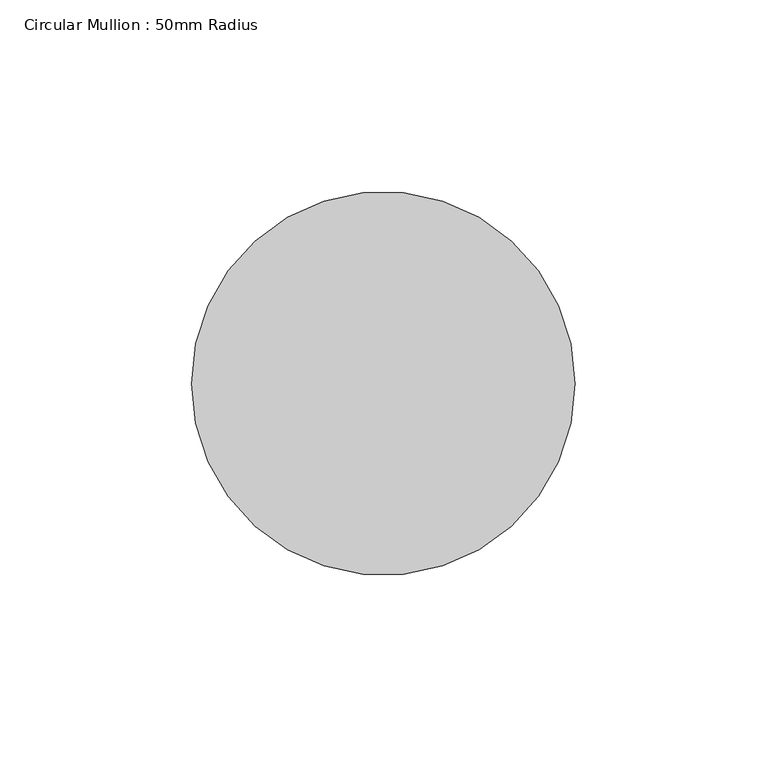
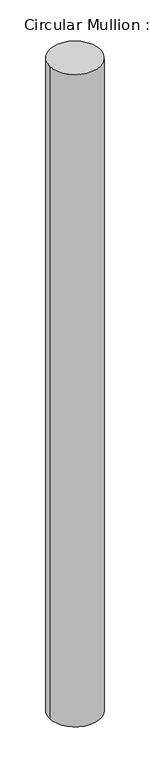
"""IFC4 building model written with IfcOpenShell, lengths in millimetres: member geometry, Circular Mullion : 50mm Radius."""

import ifcopenshell
import ifcopenshell.guid

model = None  # the IFC model being written
_history = None  # IfcOwnerHistory: only IFC2X3 demands one
_inside = {}  # id of a spatial element -> (the spatial element, [elements in it])
_under = {}  # id of a project, library or spatial element -> (it, [spatial elements below it])
_declared = {}  # id of a project -> (the project, [libraries it declares])
_typed = {}  # id of a type object -> (the type object, [elements of that type])
_made_of = {}  # id of a material, layer set ... -> (it, [elements and type objects made of it])


def new_model(schema):
    """Start an empty IFC model of exactly this schema.

    Asked for "IFC4X3", IfcOpenShell would pick the latest addendum, in which some entities
    have other attributes; the version numbers below select the first issue.
    IFC2X3 requires an IfcOwnerHistory on every rooted entity: one is made here for all.
    """
    global model, _history
    if schema == "IFC4X3":
        model = ifcopenshell.file(schema_version=(4, 3, 0, 0))
    else:
        model = ifcopenshell.file(schema=schema)
    _inside.clear()
    _under.clear()
    _declared.clear()
    _typed.clear()
    _made_of.clear()
    _history = None
    if model.schema == "IFC2X3":
        org = make("IfcOrganization", Name="unknown")
        user = make(
            "IfcPersonAndOrganization",
            ThePerson=make("IfcPerson", FamilyName="unknown"),
            TheOrganization=org,
        )
        app = make(
            "IfcApplication",
            ApplicationDeveloper=org,
            Version="unknown",
            ApplicationFullName="unknown",
            ApplicationIdentifier="unknown",
        )
        _history = make(
            "IfcOwnerHistory",
            OwningUser=user,
            OwningApplication=app,
            ChangeAction="ADDED",
            CreationDate=0,
        )
    return model


def make(cls, **values):
    """One entity of the class cls with the attributes given. An attribute that is None is left unset."""
    return model.create_entity(
        cls, **{name: value for name, value in values.items() if value is not None}
    )


def rooted(cls, **values):
    """An entity with a GlobalId (a new one), such as an element, a storey or a relation."""
    return make(cls, GlobalId=ifcopenshell.guid.new(), OwnerHistory=_history, **values)


def si_unit(unit_type, name, prefix=None):
    """IfcSIUnit, for example si_unit("LENGTHUNIT", "METRE", prefix="MILLI")."""
    return make("IfcSIUnit", UnitType=unit_type, Prefix=prefix, Name=name)


def assignment(units):
    """IfcUnitAssignment: the units of a project."""
    return None if units is None else make("IfcUnitAssignment", Units=units)


def point(xyz):
    """IfcCartesianPoint."""
    return None if xyz is None else make("IfcCartesianPoint", Coordinates=xyz)


def direction(xyz):
    """IfcDirection."""
    return None if xyz is None else make("IfcDirection", DirectionRatios=xyz)


def frame(location, z_axis=None, x_axis=None):
    """IfcAxis2Placement3D, a coordinate frame: its origin and axes. An axis left out is left unset."""
    return make(
        "IfcAxis2Placement3D",
        Location=point(location),
        Axis=direction(z_axis),
        RefDirection=direction(x_axis),
    )


def frame_2d(location, x_axis=None):
    """IfcAxis2Placement2D, a coordinate frame in the plane: its origin and x axis."""
    return make(
        "IfcAxis2Placement2D", Location=point(location), RefDirection=direction(x_axis)
    )


def origin():
    """The frame at (0, 0, 0) with its axes left unset."""
    return frame((0.0, 0.0, 0.0))


def origin_2d():
    """The frame at (0, 0) in the plane with its x axis left unset."""
    return frame_2d((0.0, 0.0))


def place(relative_to, where):
    """IfcLocalPlacement: puts the frame where relative to a parent placement (None: the world)."""
    return make(
        "IfcLocalPlacement", PlacementRelTo=relative_to, RelativePlacement=where
    )


def context(
    kind, dimensions, precision=None, world=None, true_north=None, identifier=None
):
    """IfcGeometricRepresentationContext, for example the 3D "Model" context."""
    return make(
        "IfcGeometricRepresentationContext",
        ContextIdentifier=identifier,
        ContextType=kind,
        CoordinateSpaceDimension=dimensions,
        Precision=precision,
        WorldCoordinateSystem=world,
        TrueNorth=true_north,
    )


def project(units=None, contexts=None):
    """IfcProject with its units and contexts."""
    return rooted(
        "IfcProject",
        Name="project",
        RepresentationContexts=contexts,
        UnitsInContext=assignment(units),
    )


def spatial(cls, under=None, at=None, **own):
    """A site, building, storey or space (cls), placed at a placement, below another one or the project."""
    s = rooted(cls, ObjectPlacement=at, **own)
    if under is not None:
        _under.setdefault(under.id(), (under, []))[1].append(s)
    return s


def circle_curve(where, radius):
    """IfcCircle in the frame where."""
    return make("IfcCircle", Position=where, Radius=radius)


def trimmed(basis, trim1, trim2, sense, master):
    """IfcTrimmedCurve: the piece of a basis curve between two trims."""
    return make(
        "IfcTrimmedCurve",
        BasisCurve=basis,
        Trim1=trim1,
        Trim2=trim2,
        SenseAgreement=sense,
        MasterRepresentation=master,
    )


def segment(curve, same_sense, transition):
    """IfcCompositeCurveSegment."""
    return make(
        "IfcCompositeCurveSegment",
        Transition=transition,
        SameSense=same_sense,
        ParentCurve=curve,
    )


def composite_curve(segments, self_intersect=None):
    """IfcCompositeCurve: segments joined end to end."""
    return make("IfcCompositeCurve", Segments=segments, SelfIntersect=self_intersect)


def outline(outer, holes=None, kind="AREA"):
    """IfcArbitraryClosedProfileDef: a profile drawn as a closed curve; with holes, ...WithVoids."""
    if holes is None:
        return make("IfcArbitraryClosedProfileDef", ProfileType=kind, OuterCurve=outer)
    return make(
        "IfcArbitraryProfileDefWithVoids",
        ProfileType=kind,
        OuterCurve=outer,
        InnerCurves=holes,
    )


def extrude(swept, where, along, depth):
    """IfcExtrudedAreaSolid: the profile swept, set in the frame where, extruded along a direction by depth."""
    return make(
        "IfcExtrudedAreaSolid",
        SweptArea=swept,
        Position=where,
        ExtrudedDirection=direction(along),
        Depth=depth,
    )


def shape(context_of_items, identifier, shape_type, items):
    """IfcShapeRepresentation: the items that make up one representation, for example the "Body"."""
    return make(
        "IfcShapeRepresentation",
        ContextOfItems=context_of_items,
        RepresentationIdentifier=identifier,
        RepresentationType=shape_type,
        Items=items,
    )


def source(mapping_origin, context_of_items, identifier, shape_type, items):
    """IfcRepresentationMap: a shape defined once, which mapped items show again and again."""
    return make(
        "IfcRepresentationMap",
        MappingOrigin=mapping_origin,
        MappedRepresentation=shape(context_of_items, identifier, shape_type, items),
    )


def transform(
    local_origin,
    x_axis=None,
    y_axis=None,
    z_axis=None,
    scale=None,
    scale2=None,
    scale3=None,
    uniform=True,
):
    """IfcCartesianTransformationOperator3D, or its non-uniform kind. x_axis, y_axis, z_axis: its Axis1, 2, 3."""
    if uniform:
        return make(
            "IfcCartesianTransformationOperator3D",
            Axis1=direction(x_axis),
            Axis2=direction(y_axis),
            LocalOrigin=point(local_origin),
            Scale=scale,
            Axis3=direction(z_axis),
        )
    return make(
        "IfcCartesianTransformationOperator3DnonUniform",
        Axis1=direction(x_axis),
        Axis2=direction(y_axis),
        LocalOrigin=point(local_origin),
        Scale=scale,
        Axis3=direction(z_axis),
        Scale2=scale2,
        Scale3=scale3,
    )


def mapped(mapping_source, mapping_target):
    """IfcMappedItem: shows the shape of a source again, moved by a transform."""
    return make(
        "IfcMappedItem", MappingSource=mapping_source, MappingTarget=mapping_target
    )


def made_of(thing, what):
    """Note that an element or type object is made of a material, layer set ...; save() writes the relation."""
    if what is not None:
        _made_of.setdefault(what.id(), (what, []))[1].append(thing)
    return thing


def element(
    cls,
    number,
    at=None,
    inside=None,
    cuts=None,
    type_object=None,
    material=None,
    context=None,
    identifier="Body",
    shape_type=None,
    held_by="IfcProductDefinitionShape",
    body=None,
    shapes=None,
    **own,
):
    """One element of the class cls, such as IfcWall. Its Tag is "e" and its number.

    at: its placement. inside: the storey or other place that contains it. cuts: it is an
    opening in that element (IfcRelVoidsElement). A single representation is given by context,
    identifier, shape_type and body (its items); several are given by shapes. held_by: the class
    of the entity that holds the representations. save() writes the other relations.
    """
    e = rooted(cls, Tag="e%d" % number, ObjectPlacement=at, **own)
    if body is not None:
        shapes = [shape(context, identifier, shape_type, body)]
    if shapes is not None:
        e.Representation = make(held_by, Representations=shapes)
    if inside is not None:
        _inside.setdefault(inside.id(), (inside, []))[1].append(e)
    if cuts is not None:
        rooted(
            "IfcRelVoidsElement", RelatingBuildingElement=cuts, RelatedOpeningElement=e
        )
    if type_object is not None:
        _typed.setdefault(type_object.id(), (type_object, []))[1].append(e)
    return made_of(e, material)


def aggregate(whole, parts):
    """IfcRelAggregates: a whole, such as a stair, and the parts it consists of."""
    return rooted("IfcRelAggregates", RelatingObject=whole, RelatedObjects=parts)


def save(model, path):
    """Write the relations noted so far, then the file.

    IfcRelAggregates (storeys below a building ...), IfcRelContainedInSpatialStructure (elements
    in a storey), IfcRelDefinesByType, IfcRelAssociatesMaterial and IfcRelDeclares: one each for
    every whole, place, type object, material and project.
    """
    for whole, parts in _under.values():
        aggregate(whole, parts)
    for where, things in _inside.values():
        rooted(
            "IfcRelContainedInSpatialStructure",
            RelatedElements=things,
            RelatingStructure=where,
        )
    for kind, things in _typed.values():
        rooted("IfcRelDefinesByType", RelatedObjects=things, RelatingType=kind)
    for what, things in _made_of.values():
        rooted("IfcRelAssociatesMaterial", RelatedObjects=things, RelatingMaterial=what)
    for by, libraries in _declared.values():
        rooted("IfcRelDeclares", RelatingContext=by, RelatedDefinitions=libraries)
    model.write(path)


def circular_mullion_50mm_radius_fa43af0d(model_context):
    return source(origin(), model_context, "Body", "SweptSolid", [
        extrude(outline(composite_curve([segment(trimmed(circle_curve(origin_2d(), 50.0), [point((50.0, 0.0))], [point((-50.0, 0.0))], False, "CARTESIAN"), True, "CONTINUOUS"), segment(trimmed(circle_curve(origin_2d(), 50.0), [point((-50.0, 0.0))], [point((50.0, 0.0))], False, "CARTESIAN"), True, "CONTINUOUS")], self_intersect=False)), frame((0.0, 0.0, -1361.1514537), z_axis=(0.0, 0.0, 1.0), x_axis=(1.0, 0.0, 0.0)), (0.0, 0.0, 1.0), 1361.1514537),
    ])


if __name__ == "__main__":
    model = new_model("IFC4")
    model_context = context("Model", 3, world=origin())
    ifc_project = project(units=[si_unit("LENGTHUNIT", "METRE", prefix="MILLI")], contexts=[model_context])
    site = spatial("IfcSite", under=ifc_project)
    building = spatial("IfcBuilding", under=site)
    placement = place(None, origin())
    circular_mullion_50mm_radius_shape = circular_mullion_50mm_radius_fa43af0d(model_context)
    element("IfcMember", 1, ObjectType="Circular Mullion : 50mm Radius", at=placement, inside=building, context=model_context, shape_type="MappedRepresentation", body=[
        mapped(circular_mullion_50mm_radius_shape, transform((0.0, 0.0, 0.0), x_axis=(1.0, 0.0, 0.0), y_axis=(0.0, 1.0, 0.0), z_axis=(0.0, 0.0, 1.0))),
    ])
    save(model, "model.ifc")

# Revit data of these elements
# Type "Circular Mullion : 50mm Radius"
#   built-in parameter 1007350 = 0.164042 (stored number, unit not read)
# Element 1 (IfcMember, "Circular Mullion : 50mm Radius")
#   Materials on its faces: "Aluminium"
# Materials
#   "Aluminium": class "Metal", colour RGB 247 247 247, transparency 0, Description = "Aluminium 6061", Cost = 0
